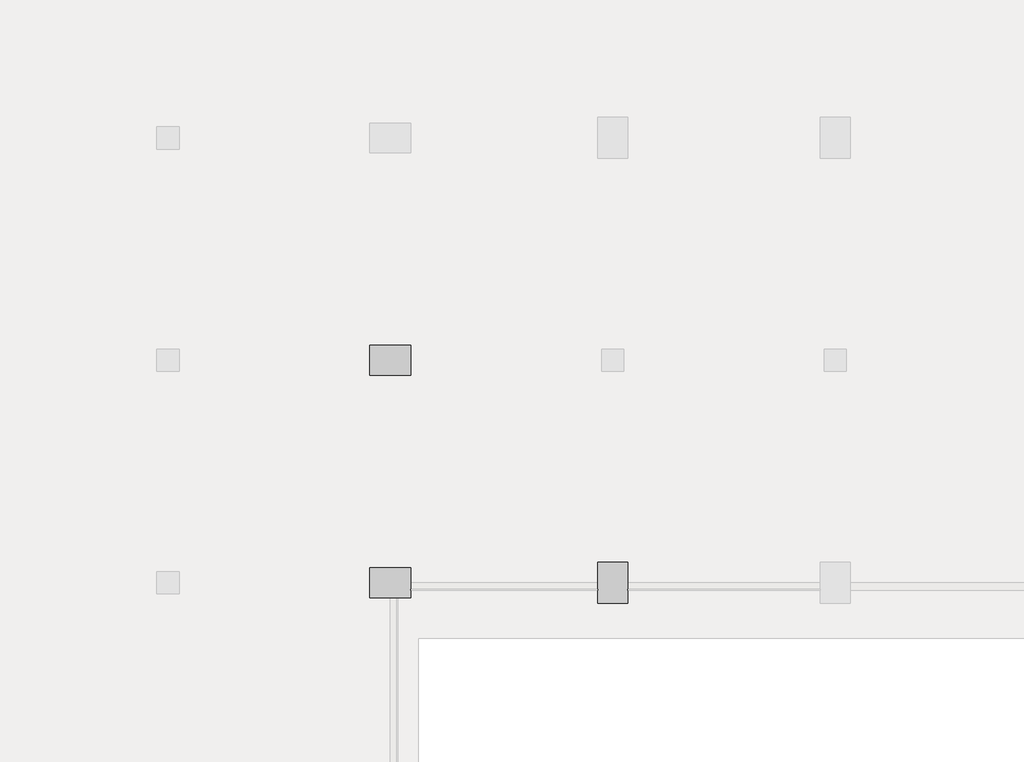
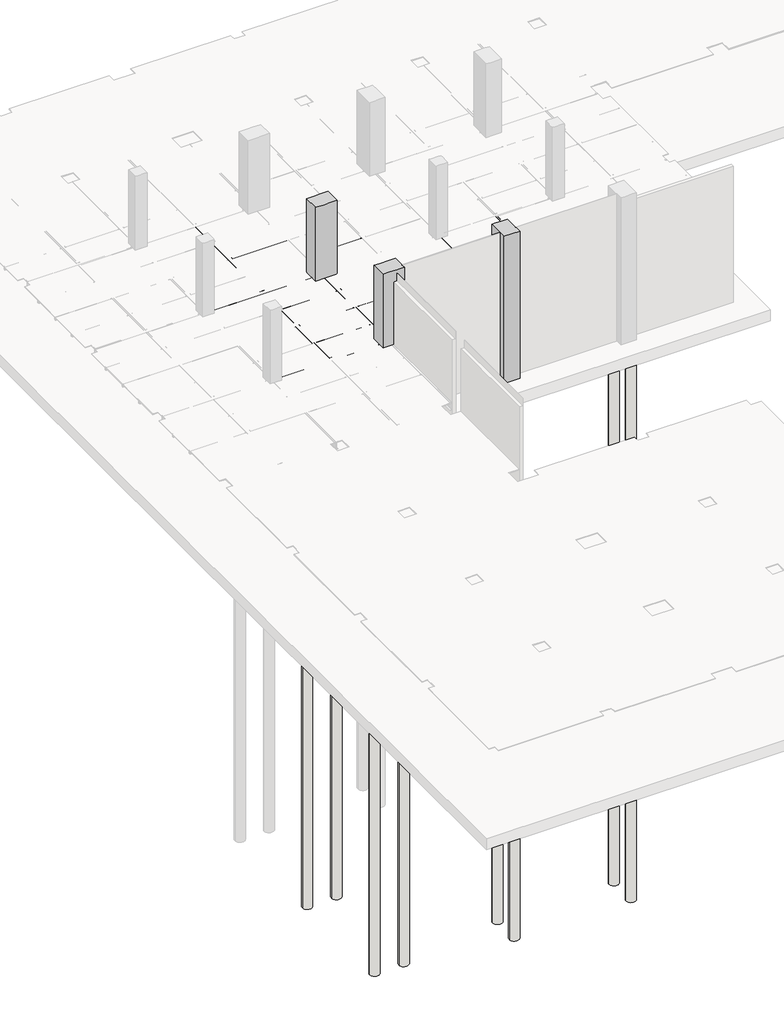
# Not in any storey, part 9 of 16: 28 beams, 8 slabs, 3 columns.
"""IFC4 building model written with IfcOpenShell, lengths in millimetres."""

from ifc_helpers import new_model, si_unit, point, frame, frame_2d, origin, place, context, project, spatial, polyline, circle_curve, trimmed, segment, composite_curve, outline, extrude, faceted_brep, element, save

model = new_model("IFC4")

# Units and contexts
model_context = context("Model", 3, world=origin())
ifc_project = project(units=[si_unit("LENGTHUNIT", "METRE", prefix="MILLI")], contexts=[model_context])

# Site, building
site = spatial("IfcSite", under=ifc_project)
building = spatial("IfcBuilding", under=site)

# Beams
placement = place(None, origin())
element("IfcBeam", 1, ObjectType="Steel Framing_H_KS : H_SB_AR_S02_H-400x200x8x13_BSG1", at=placement, inside=building, context=model_context, shape_type="SweptSolid", body=[
    extrude(outline(composite_curve([segment(polyline([(-23900.0, -4187.0381366), (-23900.0, -4200.0381366), (-24100.0, -4200.0381366), (-24100.0, -4187.0381366), (-24020.0, -4187.0381366)]), True, "CONTINUOUS"), segment(trimmed(circle_curve(frame_2d((-24020.0, -4171.0381366)), 16.0), [point((-24020.0, -4187.0381366))], [point((-24004.0, -4171.0381366))], True, "CARTESIAN"), True, "CONTINUOUS"), segment(polyline([(-24004.0, -4171.0381366), (-24004.0, -3829.0381366)]), True, "CONTINUOUS"), segment(trimmed(circle_curve(frame_2d((-24020.0, -3829.0381366)), 16.0), [point((-24004.0, -3829.0381366))], [point((-24020.0, -3813.0381366))], True, "CARTESIAN"), True, "CONTINUOUS"), segment(polyline([(-24020.0, -3813.0381366), (-24100.0, -3813.0381366), (-24100.0, -3800.0381366), (-23900.0, -3800.0381366), (-23900.0, -3813.0381366), (-23980.0, -3813.0381366)]), True, "CONTINUOUS"), segment(trimmed(circle_curve(frame_2d((-23980.0, -3829.0381366)), 16.0), [point((-23980.0, -3813.0381366))], [point((-23996.0, -3829.0381366))], True, "CARTESIAN"), True, "CONTINUOUS"), segment(polyline([(-23996.0, -3829.0381366), (-23996.0, -4171.0381366)]), True, "CONTINUOUS"), segment(trimmed(circle_curve(frame_2d((-23980.0, -4171.0381366)), 16.0), [point((-23996.0, -4171.0381366))], [point((-23980.0, -4187.0381366))], True, "CARTESIAN"), True, "CONTINUOUS"), segment(polyline([(-23980.0, -4187.0381366), (-23900.0, -4187.0381366)]), True, "CONTINUOUS")], self_intersect=False)), frame((30312.7, 0.0, 0.0), z_axis=(1.0, 0.0, 0.0), x_axis=(0.0, 1.0, 0.0)), (0.0, 0.0, 1.0), 5124.6),
])
element("IfcBeam", 2, ObjectType="Steel Framing_H_KS : H_SB_AR_S02_H-400x200x8x13_BSB1", at=placement, inside=building, context=model_context, shape_type="SweptSolid", body=[
    extrude(outline(composite_curve([segment(polyline([(-4187.0381366, 32900.0), (-4200.0381366, 32900.0), (-4200.0381366, 33100.0), (-4187.0381366, 33100.0), (-4187.0381366, 33020.0)]), True, "CONTINUOUS"), segment(trimmed(circle_curve(frame_2d((-4171.0381366, 33020.0)), 16.0), [point((-4187.0381366, 33020.0))], [point((-4171.0381366, 33004.0))], True, "CARTESIAN"), True, "CONTINUOUS"), segment(polyline([(-4171.0381366, 33004.0), (-3829.0381366, 33004.0)]), True, "CONTINUOUS"), segment(trimmed(circle_curve(frame_2d((-3829.0381366, 33020.0)), 16.0), [point((-3829.0381366, 33004.0))], [point((-3813.0381366, 33020.0))], True, "CARTESIAN"), True, "CONTINUOUS"), segment(polyline([(-3813.0381366, 33020.0), (-3813.0381366, 33100.0), (-3800.0381366, 33100.0), (-3800.0381366, 32900.0), (-3813.0381366, 32900.0), (-3813.0381366, 32980.0)]), True, "CONTINUOUS"), segment(trimmed(circle_curve(frame_2d((-3829.0381366, 32980.0)), 16.0), [point((-3813.0381366, 32980.0))], [point((-3829.0381366, 32996.0))], True, "CARTESIAN"), True, "CONTINUOUS"), segment(polyline([(-3829.0381366, 32996.0), (-4171.0381366, 32996.0)]), True, "CONTINUOUS"), segment(trimmed(circle_curve(frame_2d((-4171.0381366, 32980.0)), 16.0), [point((-4171.0381366, 32996.0))], [point((-4187.0381366, 32980.0))], True, "CARTESIAN"), True, "CONTINUOUS"), segment(polyline([(-4187.0381366, 32980.0), (-4187.0381366, 32900.0)]), True, "CONTINUOUS")], self_intersect=False)), frame((0.0, -23887.3, 0.0), z_axis=(0.0, 1.0, 0.0), x_axis=(0.0, 0.0, 1.0)), (0.0, 0.0, 1.0), 5774.6),
])
element("IfcBeam", 3, ObjectType="Steel Framing_C_KS : H_SB_AR_S02_C-150x75x6.5x10_J1", at=placement, inside=building, context=model_context, shape_type="SweptSolid", body=[
    extrude(outline(composite_curve([segment(polyline([(-20977.2, -3800.0381366), (-20977.2, -3950.0381366), (-21052.2, -3950.0381366)]), True, "CONTINUOUS"), segment(trimmed(circle_curve(frame_2d((-21042.2, -3950.0381366)), 10.0), [point((-21052.2, -3950.0381366))], [point((-21042.2, -3940.0381366))], False, "CARTESIAN"), True, "CONTINUOUS"), segment(polyline([(-21042.2, -3940.0381366), (-20983.7, -3930.7726469), (-20983.7, -3819.3036264), (-21042.2, -3810.0381366)]), True, "CONTINUOUS"), segment(trimmed(circle_curve(frame_2d((-21042.2, -3800.0381366)), 10.0), [point((-21042.2, -3810.0381366))], [point((-21052.2, -3800.0381366))], False, "CARTESIAN"), True, "CONTINUOUS"), segment(polyline([(-21052.2, -3800.0381366), (-20977.2, -3800.0381366)]), True, "CONTINUOUS")], self_intersect=False)), frame((33112.7, 0.0, 0.0), z_axis=(1.0, 0.0, 0.0), x_axis=(0.0, 1.0, 0.0)), (0.0, 0.0, 1.0), 2774.6),
])
element("IfcBeam", 4, ObjectType="Steel Framing_C_KS : H_SB_AR_S02_C-150x75x6.5x10_J1", at=placement, inside=building, context=model_context, shape_type="SweptSolid", body=[
    extrude(outline(composite_curve([segment(polyline([(-22477.2, -3800.0381366), (-22477.2, -3950.0381366), (-22552.2, -3950.0381366)]), True, "CONTINUOUS"), segment(trimmed(circle_curve(frame_2d((-22542.2, -3950.0381366)), 10.0), [point((-22552.2, -3950.0381366))], [point((-22542.2, -3940.0381366))], False, "CARTESIAN"), True, "CONTINUOUS"), segment(polyline([(-22542.2, -3940.0381366), (-22483.7, -3930.7726469), (-22483.7, -3819.3036264), (-22542.2, -3810.0381366)]), True, "CONTINUOUS"), segment(trimmed(circle_curve(frame_2d((-22542.2, -3800.0381366)), 10.0), [point((-22542.2, -3810.0381366))], [point((-22552.2, -3800.0381366))], False, "CARTESIAN"), True, "CONTINUOUS"), segment(polyline([(-22552.2, -3800.0381366), (-22477.2, -3800.0381366)]), True, "CONTINUOUS")], self_intersect=False)), frame((33112.7, 0.0, 0.0), z_axis=(1.0, 0.0, 0.0), x_axis=(0.0, 1.0, 0.0)), (0.0, 0.0, 1.0), 2774.6),
])
element("IfcBeam", 5, ObjectType="Steel Framing_C_KS : H_SB_AR_S02_C-150x75x6.5x10_J1", at=placement, inside=building, context=model_context, shape_type="SweptSolid", body=[
    extrude(outline(composite_curve([segment(polyline([(-22477.2, -3800.0381366), (-22477.2, -3950.0381366), (-22552.2, -3950.0381366)]), True, "CONTINUOUS"), segment(trimmed(circle_curve(frame_2d((-22542.2, -3950.0381366)), 10.0), [point((-22552.2, -3950.0381366))], [point((-22542.2, -3940.0381366))], False, "CARTESIAN"), True, "CONTINUOUS"), segment(polyline([(-22542.2, -3940.0381366), (-22483.7, -3930.7726469), (-22483.7, -3819.3036264), (-22542.2, -3810.0381366)]), True, "CONTINUOUS"), segment(trimmed(circle_curve(frame_2d((-22542.2, -3800.0381366)), 10.0), [point((-22542.2, -3810.0381366))], [point((-22552.2, -3800.0381366))], False, "CARTESIAN"), True, "CONTINUOUS"), segment(polyline([(-22552.2, -3800.0381366), (-22477.2, -3800.0381366)]), True, "CONTINUOUS")], self_intersect=False)), frame((36112.7, 0.0, 0.0), z_axis=(1.0, 0.0, 0.0), x_axis=(0.0, 1.0, 0.0)), (0.0, 0.0, 1.0), 2774.6),
])
element("IfcBeam", 6, ObjectType="Steel Framing_H_KS : H_SB_AR_S02_H-400x200x8x13_BSG1", at=placement, inside=building, context=model_context, shape_type="SweptSolid", body=[
    extrude(outline(composite_curve([segment(polyline([(-29900.0, -4187.0381366), (-29900.0, -4200.0381366), (-30100.0, -4200.0381366), (-30100.0, -4187.0381366), (-30020.0, -4187.0381366)]), True, "CONTINUOUS"), segment(trimmed(circle_curve(frame_2d((-30020.0, -4171.0381366)), 16.0), [point((-30020.0, -4187.0381366))], [point((-30004.0, -4171.0381366))], True, "CARTESIAN"), True, "CONTINUOUS"), segment(polyline([(-30004.0, -4171.0381366), (-30004.0, -3829.0381366)]), True, "CONTINUOUS"), segment(trimmed(circle_curve(frame_2d((-30020.0, -3829.0381366)), 16.0), [point((-30004.0, -3829.0381366))], [point((-30020.0, -3813.0381366))], True, "CARTESIAN"), True, "CONTINUOUS"), segment(polyline([(-30020.0, -3813.0381366), (-30100.0, -3813.0381366), (-30100.0, -3800.0381366), (-29900.0, -3800.0381366), (-29900.0, -3813.0381366), (-29980.0, -3813.0381366)]), True, "CONTINUOUS"), segment(trimmed(circle_curve(frame_2d((-29980.0, -3829.0381366)), 16.0), [point((-29980.0, -3813.0381366))], [point((-29996.0, -3829.0381366))], True, "CARTESIAN"), True, "CONTINUOUS"), segment(polyline([(-29996.0, -3829.0381366), (-29996.0, -4171.0381366)]), True, "CONTINUOUS"), segment(trimmed(circle_curve(frame_2d((-29980.0, -4171.0381366)), 16.0), [point((-29996.0, -4171.0381366))], [point((-29980.0, -4187.0381366))], True, "CARTESIAN"), True, "CONTINUOUS"), segment(polyline([(-29980.0, -4187.0381366), (-29900.0, -4187.0381366)]), True, "CONTINUOUS")], self_intersect=False)), frame((30312.7, 0.0, 0.0), z_axis=(1.0, 0.0, 0.0), x_axis=(0.0, 1.0, 0.0)), (0.0, 0.0, 1.0), 5124.6),
])
element("IfcBeam", 7, ObjectType="Steel Framing_H_KS : H_SB_AR_S02_H-400x200x8x13_BSG2", at=placement, inside=building, context=model_context, shape_type="SweptSolid", body=[
    extrude(outline(composite_curve([segment(polyline([(-4187.0381366, 35900.0), (-4200.0381366, 35900.0), (-4200.0381366, 36100.0), (-4187.0381366, 36100.0), (-4187.0381366, 36020.0)]), True, "CONTINUOUS"), segment(trimmed(circle_curve(frame_2d((-4171.0381366, 36020.0)), 16.0), [point((-4187.0381366, 36020.0))], [point((-4171.0381366, 36004.0))], True, "CARTESIAN"), True, "CONTINUOUS"), segment(polyline([(-4171.0381366, 36004.0), (-3829.0381366, 36004.0)]), True, "CONTINUOUS"), segment(trimmed(circle_curve(frame_2d((-3829.0381366, 36020.0)), 16.0), [point((-3829.0381366, 36004.0))], [point((-3813.0381366, 36020.0))], True, "CARTESIAN"), True, "CONTINUOUS"), segment(polyline([(-3813.0381366, 36020.0), (-3813.0381366, 36100.0), (-3800.0381366, 36100.0), (-3800.0381366, 35900.0), (-3813.0381366, 35900.0), (-3813.0381366, 35980.0)]), True, "CONTINUOUS"), segment(trimmed(circle_curve(frame_2d((-3829.0381366, 35980.0)), 16.0), [point((-3813.0381366, 35980.0))], [point((-3829.0381366, 35996.0))], True, "CARTESIAN"), True, "CONTINUOUS"), segment(polyline([(-3829.0381366, 35996.0), (-4171.0381366, 35996.0)]), True, "CONTINUOUS"), segment(trimmed(circle_curve(frame_2d((-4171.0381366, 35980.0)), 16.0), [point((-4171.0381366, 35996.0))], [point((-4187.0381366, 35980.0))], True, "CARTESIAN"), True, "CONTINUOUS"), segment(polyline([(-4187.0381366, 35980.0), (-4187.0381366, 35900.0)]), True, "CONTINUOUS")], self_intersect=False)), frame((0.0, -29587.3, 0.0), z_axis=(0.0, 1.0, 0.0), x_axis=(0.0, 0.0, 1.0)), (0.0, 0.0, 1.0), 5174.6),
])
element("IfcBeam", 8, ObjectType="Steel Framing_H_KS : H_SB_AR_S02_H-400x200x8x13_BSB1", at=placement, inside=building, context=model_context, shape_type="SweptSolid", body=[
    extrude(outline(composite_curve([segment(polyline([(-4187.0381366, 32900.0), (-4200.0381366, 32900.0), (-4200.0381366, 33100.0), (-4187.0381366, 33100.0), (-4187.0381366, 33020.0)]), True, "CONTINUOUS"), segment(trimmed(circle_curve(frame_2d((-4171.0381366, 33020.0)), 16.0), [point((-4187.0381366, 33020.0))], [point((-4171.0381366, 33004.0))], True, "CARTESIAN"), True, "CONTINUOUS"), segment(polyline([(-4171.0381366, 33004.0), (-3829.0381366, 33004.0)]), True, "CONTINUOUS"), segment(trimmed(circle_curve(frame_2d((-3829.0381366, 33020.0)), 16.0), [point((-3829.0381366, 33004.0))], [point((-3813.0381366, 33020.0))], True, "CARTESIAN"), True, "CONTINUOUS"), segment(polyline([(-3813.0381366, 33020.0), (-3813.0381366, 33100.0), (-3800.0381366, 33100.0), (-3800.0381366, 32900.0), (-3813.0381366, 32900.0), (-3813.0381366, 32980.0)]), True, "CONTINUOUS"), segment(trimmed(circle_curve(frame_2d((-3829.0381366, 32980.0)), 16.0), [point((-3813.0381366, 32980.0))], [point((-3829.0381366, 32996.0))], True, "CARTESIAN"), True, "CONTINUOUS"), segment(polyline([(-3829.0381366, 32996.0), (-4171.0381366, 32996.0)]), True, "CONTINUOUS"), segment(trimmed(circle_curve(frame_2d((-4171.0381366, 32980.0)), 16.0), [point((-4171.0381366, 32996.0))], [point((-4187.0381366, 32980.0))], True, "CARTESIAN"), True, "CONTINUOUS"), segment(polyline([(-4187.0381366, 32980.0), (-4187.0381366, 32900.0)]), True, "CONTINUOUS")], self_intersect=False)), frame((0.0, -29887.3, 0.0), z_axis=(0.0, 1.0, 0.0), x_axis=(0.0, 0.0, 1.0)), (0.0, 0.0, 1.0), 5774.6),
])
element("IfcBeam", 9, ObjectType="Steel Framing_C_KS : H_SB_AR_S02_C-150x75x6.5x10_J1", at=placement, inside=building, context=model_context, shape_type="SweptSolid", body=[
    extrude(outline(composite_curve([segment(polyline([(-26977.2, -3800.0381366), (-26977.2, -3950.0381366), (-27052.2, -3950.0381366)]), True, "CONTINUOUS"), segment(trimmed(circle_curve(frame_2d((-27042.2, -3950.0381366)), 10.0), [point((-27052.2, -3950.0381366))], [point((-27042.2, -3940.0381366))], False, "CARTESIAN"), True, "CONTINUOUS"), segment(polyline([(-27042.2, -3940.0381366), (-26983.7, -3930.7726469), (-26983.7, -3819.3036264), (-27042.2, -3810.0381366)]), True, "CONTINUOUS"), segment(trimmed(circle_curve(frame_2d((-27042.2, -3800.0381366)), 10.0), [point((-27042.2, -3810.0381366))], [point((-27052.2, -3800.0381366))], False, "CARTESIAN"), True, "CONTINUOUS"), segment(polyline([(-27052.2, -3800.0381366), (-26977.2, -3800.0381366)]), True, "CONTINUOUS")], self_intersect=False)), frame((33112.7, 0.0, 0.0), z_axis=(1.0, 0.0, 0.0), x_axis=(0.0, 1.0, 0.0)), (0.0, 0.0, 1.0), 2774.6),
])
element("IfcBeam", 10, ObjectType="Steel Framing_C_KS : H_SB_AR_S02_C-150x75x6.5x10_J1", at=placement, inside=building, context=model_context, shape_type="SweptSolid", body=[
    extrude(outline(composite_curve([segment(polyline([(-28477.2, -3800.0381366), (-28477.2, -3950.0381366), (-28552.2, -3950.0381366)]), True, "CONTINUOUS"), segment(trimmed(circle_curve(frame_2d((-28542.2, -3950.0381366)), 10.0), [point((-28552.2, -3950.0381366))], [point((-28542.2, -3940.0381366))], False, "CARTESIAN"), True, "CONTINUOUS"), segment(polyline([(-28542.2, -3940.0381366), (-28483.7, -3930.7726469), (-28483.7, -3819.3036264), (-28542.2, -3810.0381366)]), True, "CONTINUOUS"), segment(trimmed(circle_curve(frame_2d((-28542.2, -3800.0381366)), 10.0), [point((-28542.2, -3810.0381366))], [point((-28552.2, -3800.0381366))], False, "CARTESIAN"), True, "CONTINUOUS"), segment(polyline([(-28552.2, -3800.0381366), (-28477.2, -3800.0381366)]), True, "CONTINUOUS")], self_intersect=False)), frame((33112.7, 0.0, 0.0), z_axis=(1.0, 0.0, 0.0), x_axis=(0.0, 1.0, 0.0)), (0.0, 0.0, 1.0), 2774.6),
])
element("IfcBeam", 11, ObjectType="Steel Framing_C_KS : H_SB_AR_S02_C-150x75x6.5x10_J1", at=placement, inside=building, context=model_context, shape_type="SweptSolid", body=[
    extrude(outline(composite_curve([segment(polyline([(-25477.2, -3800.0381366), (-25477.2, -3950.0381366), (-25552.2, -3950.0381366)]), True, "CONTINUOUS"), segment(trimmed(circle_curve(frame_2d((-25542.2, -3950.0381366)), 10.0), [point((-25552.2, -3950.0381366))], [point((-25542.2, -3940.0381366))], False, "CARTESIAN"), True, "CONTINUOUS"), segment(polyline([(-25542.2, -3940.0381366), (-25483.7, -3930.7726469), (-25483.7, -3819.3036264), (-25542.2, -3810.0381366)]), True, "CONTINUOUS"), segment(trimmed(circle_curve(frame_2d((-25542.2, -3800.0381366)), 10.0), [point((-25542.2, -3810.0381366))], [point((-25552.2, -3800.0381366))], False, "CARTESIAN"), True, "CONTINUOUS"), segment(polyline([(-25552.2, -3800.0381366), (-25477.2, -3800.0381366)]), True, "CONTINUOUS")], self_intersect=False)), frame((33112.7, 0.0, 0.0), z_axis=(1.0, 0.0, 0.0), x_axis=(0.0, 1.0, 0.0)), (0.0, 0.0, 1.0), 2774.6),
])
element("IfcBeam", 12, ObjectType="Steel Framing_H_KS : H_SB_AR_S02_H-400x200x8x13_BSG1", at=placement, inside=building, context=model_context, shape_type="SweptSolid", body=[
    extrude(outline(composite_curve([segment(polyline([(-29900.0, -4187.0381366), (-29900.0, -4200.0381366), (-30100.0, -4200.0381366), (-30100.0, -4187.0381366), (-30020.0, -4187.0381366)]), True, "CONTINUOUS"), segment(trimmed(circle_curve(frame_2d((-30020.0, -4171.0381366)), 16.0), [point((-30020.0, -4187.0381366))], [point((-30004.0, -4171.0381366))], True, "CARTESIAN"), True, "CONTINUOUS"), segment(polyline([(-30004.0, -4171.0381366), (-30004.0, -3829.0381366)]), True, "CONTINUOUS"), segment(trimmed(circle_curve(frame_2d((-30020.0, -3829.0381366)), 16.0), [point((-30004.0, -3829.0381366))], [point((-30020.0, -3813.0381366))], True, "CARTESIAN"), True, "CONTINUOUS"), segment(polyline([(-30020.0, -3813.0381366), (-30100.0, -3813.0381366), (-30100.0, -3800.0381366), (-29900.0, -3800.0381366), (-29900.0, -3813.0381366), (-29980.0, -3813.0381366)]), True, "CONTINUOUS"), segment(trimmed(circle_curve(frame_2d((-29980.0, -3829.0381366)), 16.0), [point((-29980.0, -3813.0381366))], [point((-29996.0, -3829.0381366))], True, "CARTESIAN"), True, "CONTINUOUS"), segment(polyline([(-29996.0, -3829.0381366), (-29996.0, -4171.0381366)]), True, "CONTINUOUS"), segment(trimmed(circle_curve(frame_2d((-29980.0, -4171.0381366)), 16.0), [point((-29996.0, -4171.0381366))], [point((-29980.0, -4187.0381366))], True, "CARTESIAN"), True, "CONTINUOUS"), segment(polyline([(-29980.0, -4187.0381366), (-29900.0, -4187.0381366)]), True, "CONTINUOUS")], self_intersect=False)), frame((36562.7, 0.0, 0.0), z_axis=(1.0, 0.0, 0.0), x_axis=(0.0, 1.0, 0.0)), (0.0, 0.0, 1.0), 5024.6),
])
element("IfcBeam", 13, ObjectType="Steel Framing_H_KS : H_SB_AR_S02_H-400x200x8x13_BSG2", at=placement, inside=building, context=model_context, shape_type="SweptSolid", body=[
    extrude(outline(composite_curve([segment(polyline([(-4187.0381366, 41900.0), (-4200.0381366, 41900.0), (-4200.0381366, 42100.0), (-4187.0381366, 42100.0), (-4187.0381366, 42020.0)]), True, "CONTINUOUS"), segment(trimmed(circle_curve(frame_2d((-4171.0381366, 42020.0)), 16.0), [point((-4187.0381366, 42020.0))], [point((-4171.0381366, 42004.0))], True, "CARTESIAN"), True, "CONTINUOUS"), segment(polyline([(-4171.0381366, 42004.0), (-3829.0381366, 42004.0)]), True, "CONTINUOUS"), segment(trimmed(circle_curve(frame_2d((-3829.0381366, 42020.0)), 16.0), [point((-3829.0381366, 42004.0))], [point((-3813.0381366, 42020.0))], True, "CARTESIAN"), True, "CONTINUOUS"), segment(polyline([(-3813.0381366, 42020.0), (-3813.0381366, 42100.0), (-3800.0381366, 42100.0), (-3800.0381366, 41900.0), (-3813.0381366, 41900.0), (-3813.0381366, 41980.0)]), True, "CONTINUOUS"), segment(trimmed(circle_curve(frame_2d((-3829.0381366, 41980.0)), 16.0), [point((-3813.0381366, 41980.0))], [point((-3829.0381366, 41996.0))], True, "CARTESIAN"), True, "CONTINUOUS"), segment(polyline([(-3829.0381366, 41996.0), (-4171.0381366, 41996.0)]), True, "CONTINUOUS"), segment(trimmed(circle_curve(frame_2d((-4171.0381366, 41980.0)), 16.0), [point((-4171.0381366, 41996.0))], [point((-4187.0381366, 41980.0))], True, "CARTESIAN"), True, "CONTINUOUS"), segment(polyline([(-4187.0381366, 41980.0), (-4187.0381366, 41900.0)]), True, "CONTINUOUS")], self_intersect=False)), frame((0.0, -29437.3, 0.0), z_axis=(0.0, 1.0, 0.0), x_axis=(0.0, 0.0, 1.0)), (0.0, 0.0, 1.0), 5124.6),
])
element("IfcBeam", 14, ObjectType="Steel Framing_H_KS : H_SB_AR_S02_H-400x200x8x13_BSB1", at=placement, inside=building, context=model_context, shape_type="SweptSolid", body=[
    extrude(outline(composite_curve([segment(polyline([(-4187.0381366, 38900.0), (-4200.0381366, 38900.0), (-4200.0381366, 39100.0), (-4187.0381366, 39100.0), (-4187.0381366, 39020.0)]), True, "CONTINUOUS"), segment(trimmed(circle_curve(frame_2d((-4171.0381366, 39020.0)), 16.0), [point((-4187.0381366, 39020.0))], [point((-4171.0381366, 39004.0))], True, "CARTESIAN"), True, "CONTINUOUS"), segment(polyline([(-4171.0381366, 39004.0), (-3829.0381366, 39004.0)]), True, "CONTINUOUS"), segment(trimmed(circle_curve(frame_2d((-3829.0381366, 39020.0)), 16.0), [point((-3829.0381366, 39004.0))], [point((-3813.0381366, 39020.0))], True, "CARTESIAN"), True, "CONTINUOUS"), segment(polyline([(-3813.0381366, 39020.0), (-3813.0381366, 39100.0), (-3800.0381366, 39100.0), (-3800.0381366, 38900.0), (-3813.0381366, 38900.0), (-3813.0381366, 38980.0)]), True, "CONTINUOUS"), segment(trimmed(circle_curve(frame_2d((-3829.0381366, 38980.0)), 16.0), [point((-3813.0381366, 38980.0))], [point((-3829.0381366, 38996.0))], True, "CARTESIAN"), True, "CONTINUOUS"), segment(polyline([(-3829.0381366, 38996.0), (-4171.0381366, 38996.0)]), True, "CONTINUOUS"), segment(trimmed(circle_curve(frame_2d((-4171.0381366, 38980.0)), 16.0), [point((-4171.0381366, 38996.0))], [point((-4187.0381366, 38980.0))], True, "CARTESIAN"), True, "CONTINUOUS"), segment(polyline([(-4187.0381366, 38980.0), (-4187.0381366, 38900.0)]), True, "CONTINUOUS")], self_intersect=False)), frame((0.0, -29887.3, 0.0), z_axis=(0.0, 1.0, 0.0), x_axis=(0.0, 0.0, 1.0)), (0.0, 0.0, 1.0), 5774.6),
])
element("IfcBeam", 15, ObjectType="Steel Framing_C_KS : H_SB_AR_S02_C-150x75x6.5x10_J1", at=placement, inside=building, context=model_context, shape_type="SweptSolid", body=[
    extrude(outline(composite_curve([segment(polyline([(-26977.2, -3800.0381366), (-26977.2, -3950.0381366), (-27052.2, -3950.0381366)]), True, "CONTINUOUS"), segment(trimmed(circle_curve(frame_2d((-27042.2, -3950.0381366)), 10.0), [point((-27052.2, -3950.0381366))], [point((-27042.2, -3940.0381366))], False, "CARTESIAN"), True, "CONTINUOUS"), segment(polyline([(-27042.2, -3940.0381366), (-26983.7, -3930.7726469), (-26983.7, -3819.3036264), (-27042.2, -3810.0381366)]), True, "CONTINUOUS"), segment(trimmed(circle_curve(frame_2d((-27042.2, -3800.0381366)), 10.0), [point((-27042.2, -3810.0381366))], [point((-27052.2, -3800.0381366))], False, "CARTESIAN"), True, "CONTINUOUS"), segment(polyline([(-27052.2, -3800.0381366), (-26977.2, -3800.0381366)]), True, "CONTINUOUS")], self_intersect=False)), frame((36112.7, 0.0, 0.0), z_axis=(1.0, 0.0, 0.0), x_axis=(0.0, 1.0, 0.0)), (0.0, 0.0, 1.0), 2774.6),
])
element("IfcBeam", 16, ObjectType="Steel Framing_C_KS : H_SB_AR_S02_C-150x75x6.5x10_J1", at=placement, inside=building, context=model_context, shape_type="SweptSolid", body=[
    extrude(outline(composite_curve([segment(polyline([(-28477.2, -3800.0381366), (-28477.2, -3950.0381366), (-28552.2, -3950.0381366)]), True, "CONTINUOUS"), segment(trimmed(circle_curve(frame_2d((-28542.2, -3950.0381366)), 10.0), [point((-28552.2, -3950.0381366))], [point((-28542.2, -3940.0381366))], False, "CARTESIAN"), True, "CONTINUOUS"), segment(polyline([(-28542.2, -3940.0381366), (-28483.7, -3930.7726469), (-28483.7, -3819.3036264), (-28542.2, -3810.0381366)]), True, "CONTINUOUS"), segment(trimmed(circle_curve(frame_2d((-28542.2, -3800.0381366)), 10.0), [point((-28542.2, -3810.0381366))], [point((-28552.2, -3800.0381366))], False, "CARTESIAN"), True, "CONTINUOUS"), segment(polyline([(-28552.2, -3800.0381366), (-28477.2, -3800.0381366)]), True, "CONTINUOUS")], self_intersect=False)), frame((36112.7, 0.0, 0.0), z_axis=(1.0, 0.0, 0.0), x_axis=(0.0, 1.0, 0.0)), (0.0, 0.0, 1.0), 2774.6),
])
element("IfcBeam", 17, ObjectType="Steel Framing_C_KS : H_SB_AR_S02_C-150x75x6.5x10_J1", at=placement, inside=building, context=model_context, shape_type="SweptSolid", body=[
    extrude(outline(composite_curve([segment(polyline([(-25477.2, -3800.0381366), (-25477.2, -3950.0381366), (-25552.2, -3950.0381366)]), True, "CONTINUOUS"), segment(trimmed(circle_curve(frame_2d((-25542.2, -3950.0381366)), 10.0), [point((-25552.2, -3950.0381366))], [point((-25542.2, -3940.0381366))], False, "CARTESIAN"), True, "CONTINUOUS"), segment(polyline([(-25542.2, -3940.0381366), (-25483.7, -3930.7726469), (-25483.7, -3819.3036264), (-25542.2, -3810.0381366)]), True, "CONTINUOUS"), segment(trimmed(circle_curve(frame_2d((-25542.2, -3800.0381366)), 10.0), [point((-25542.2, -3810.0381366))], [point((-25552.2, -3800.0381366))], False, "CARTESIAN"), True, "CONTINUOUS"), segment(polyline([(-25552.2, -3800.0381366), (-25477.2, -3800.0381366)]), True, "CONTINUOUS")], self_intersect=False)), frame((36112.7, 0.0, 0.0), z_axis=(1.0, 0.0, 0.0), x_axis=(0.0, 1.0, 0.0)), (0.0, 0.0, 1.0), 2774.6),
])
element("IfcBeam", 18, ObjectType="Steel Framing_C_KS : H_SB_AR_S02_C-150x75x6.5x10_J1", at=placement, inside=building, context=model_context, shape_type="SweptSolid", body=[
    extrude(outline(composite_curve([segment(polyline([(-26977.2, -3800.0381366), (-26977.2, -3950.0381366), (-27052.2, -3950.0381366)]), True, "CONTINUOUS"), segment(trimmed(circle_curve(frame_2d((-27042.2, -3950.0381366)), 10.0), [point((-27052.2, -3950.0381366))], [point((-27042.2, -3940.0381366))], False, "CARTESIAN"), True, "CONTINUOUS"), segment(polyline([(-27042.2, -3940.0381366), (-26983.7, -3930.7726469), (-26983.7, -3819.3036264), (-27042.2, -3810.0381366)]), True, "CONTINUOUS"), segment(trimmed(circle_curve(frame_2d((-27042.2, -3800.0381366)), 10.0), [point((-27042.2, -3810.0381366))], [point((-27052.2, -3800.0381366))], False, "CARTESIAN"), True, "CONTINUOUS"), segment(polyline([(-27052.2, -3800.0381366), (-26977.2, -3800.0381366)]), True, "CONTINUOUS")], self_intersect=False)), frame((39112.7, 0.0, 0.0), z_axis=(1.0, 0.0, 0.0), x_axis=(0.0, 1.0, 0.0)), (0.0, 0.0, 1.0), 2774.6),
])
element("IfcBeam", 19, ObjectType="Steel Framing_C_KS : H_SB_AR_S02_C-150x75x6.5x10_J1", at=placement, inside=building, context=model_context, shape_type="SweptSolid", body=[
    extrude(outline(composite_curve([segment(polyline([(-28477.2, -3800.0381366), (-28477.2, -3950.0381366), (-28552.2, -3950.0381366)]), True, "CONTINUOUS"), segment(trimmed(circle_curve(frame_2d((-28542.2, -3950.0381366)), 10.0), [point((-28552.2, -3950.0381366))], [point((-28542.2, -3940.0381366))], False, "CARTESIAN"), True, "CONTINUOUS"), segment(polyline([(-28542.2, -3940.0381366), (-28483.7, -3930.7726469), (-28483.7, -3819.3036264), (-28542.2, -3810.0381366)]), True, "CONTINUOUS"), segment(trimmed(circle_curve(frame_2d((-28542.2, -3800.0381366)), 10.0), [point((-28542.2, -3810.0381366))], [point((-28552.2, -3800.0381366))], False, "CARTESIAN"), True, "CONTINUOUS"), segment(polyline([(-28552.2, -3800.0381366), (-28477.2, -3800.0381366)]), True, "CONTINUOUS")], self_intersect=False)), frame((39112.7, 0.0, 0.0), z_axis=(1.0, 0.0, 0.0), x_axis=(0.0, 1.0, 0.0)), (0.0, 0.0, 1.0), 2774.6),
])
element("IfcBeam", 20, ObjectType="Steel Framing_C_KS : H_SB_AR_S02_C-150x75x6.5x10_J1", at=placement, inside=building, context=model_context, shape_type="SweptSolid", body=[
    extrude(outline(composite_curve([segment(polyline([(-25477.2, -3800.0381366), (-25477.2, -3950.0381366), (-25552.2, -3950.0381366)]), True, "CONTINUOUS"), segment(trimmed(circle_curve(frame_2d((-25542.2, -3950.0381366)), 10.0), [point((-25552.2, -3950.0381366))], [point((-25542.2, -3940.0381366))], False, "CARTESIAN"), True, "CONTINUOUS"), segment(polyline([(-25542.2, -3940.0381366), (-25483.7, -3930.7726469), (-25483.7, -3819.3036264), (-25542.2, -3810.0381366)]), True, "CONTINUOUS"), segment(trimmed(circle_curve(frame_2d((-25542.2, -3800.0381366)), 10.0), [point((-25542.2, -3810.0381366))], [point((-25552.2, -3800.0381366))], False, "CARTESIAN"), True, "CONTINUOUS"), segment(polyline([(-25552.2, -3800.0381366), (-25477.2, -3800.0381366)]), True, "CONTINUOUS")], self_intersect=False)), frame((39112.7, 0.0, 0.0), z_axis=(1.0, 0.0, 0.0), x_axis=(0.0, 1.0, 0.0)), (0.0, 0.0, 1.0), 2774.6),
])
element("IfcBeam", 21, ObjectType="Steel Framing_H_KS : H_SB_AR_S02_H-400x200x8x13_BSG1", at=placement, inside=building, context=model_context, shape_type="SweptSolid", body=[
    extrude(outline(composite_curve([segment(polyline([(-29900.0, -4187.0381366), (-29900.0, -4200.0381366), (-30100.0, -4200.0381366), (-30100.0, -4187.0381366), (-30020.0, -4187.0381366)]), True, "CONTINUOUS"), segment(trimmed(circle_curve(frame_2d((-30020.0, -4171.0381366)), 16.0), [point((-30020.0, -4187.0381366))], [point((-30004.0, -4171.0381366))], True, "CARTESIAN"), True, "CONTINUOUS"), segment(polyline([(-30004.0, -4171.0381366), (-30004.0, -3829.0381366)]), True, "CONTINUOUS"), segment(trimmed(circle_curve(frame_2d((-30020.0, -3829.0381366)), 16.0), [point((-30004.0, -3829.0381366))], [point((-30020.0, -3813.0381366))], True, "CARTESIAN"), True, "CONTINUOUS"), segment(polyline([(-30020.0, -3813.0381366), (-30100.0, -3813.0381366), (-30100.0, -3800.0381366), (-29900.0, -3800.0381366), (-29900.0, -3813.0381366), (-29980.0, -3813.0381366)]), True, "CONTINUOUS"), segment(trimmed(circle_curve(frame_2d((-29980.0, -3829.0381366)), 16.0), [point((-29980.0, -3813.0381366))], [point((-29996.0, -3829.0381366))], True, "CARTESIAN"), True, "CONTINUOUS"), segment(polyline([(-29996.0, -3829.0381366), (-29996.0, -4171.0381366)]), True, "CONTINUOUS"), segment(trimmed(circle_curve(frame_2d((-29980.0, -4171.0381366)), 16.0), [point((-29996.0, -4171.0381366))], [point((-29980.0, -4187.0381366))], True, "CARTESIAN"), True, "CONTINUOUS"), segment(polyline([(-29980.0, -4187.0381366), (-29900.0, -4187.0381366)]), True, "CONTINUOUS")], self_intersect=False)), frame((42412.7, 0.0, 0.0), z_axis=(1.0, 0.0, 0.0), x_axis=(0.0, 1.0, 0.0)), (0.0, 0.0, 1.0), 5174.6),
])
element("IfcBeam", 22, ObjectType="Steel Framing_H_KS : H_SB_AR_S02_H-400x200x8x13_BSB1", at=placement, inside=building, context=model_context, shape_type="SweptSolid", body=[
    extrude(outline(composite_curve([segment(polyline([(-4187.0381366, 44900.0), (-4200.0381366, 44900.0), (-4200.0381366, 45100.0), (-4187.0381366, 45100.0), (-4187.0381366, 45020.0)]), True, "CONTINUOUS"), segment(trimmed(circle_curve(frame_2d((-4171.0381366, 45020.0)), 16.0), [point((-4187.0381366, 45020.0))], [point((-4171.0381366, 45004.0))], True, "CARTESIAN"), True, "CONTINUOUS"), segment(polyline([(-4171.0381366, 45004.0), (-3829.0381366, 45004.0)]), True, "CONTINUOUS"), segment(trimmed(circle_curve(frame_2d((-3829.0381366, 45020.0)), 16.0), [point((-3829.0381366, 45004.0))], [point((-3813.0381366, 45020.0))], True, "CARTESIAN"), True, "CONTINUOUS"), segment(polyline([(-3813.0381366, 45020.0), (-3813.0381366, 45100.0), (-3800.0381366, 45100.0), (-3800.0381366, 44900.0), (-3813.0381366, 44900.0), (-3813.0381366, 44980.0)]), True, "CONTINUOUS"), segment(trimmed(circle_curve(frame_2d((-3829.0381366, 44980.0)), 16.0), [point((-3813.0381366, 44980.0))], [point((-3829.0381366, 44996.0))], True, "CARTESIAN"), True, "CONTINUOUS"), segment(polyline([(-3829.0381366, 44996.0), (-4171.0381366, 44996.0)]), True, "CONTINUOUS"), segment(trimmed(circle_curve(frame_2d((-4171.0381366, 44980.0)), 16.0), [point((-4171.0381366, 44996.0))], [point((-4187.0381366, 44980.0))], True, "CARTESIAN"), True, "CONTINUOUS"), segment(polyline([(-4187.0381366, 44980.0), (-4187.0381366, 44900.0)]), True, "CONTINUOUS")], self_intersect=False)), frame((0.0, -29887.3, 0.0), z_axis=(0.0, 1.0, 0.0), x_axis=(0.0, 0.0, 1.0)), (0.0, 0.0, 1.0), 5774.6),
])
element("IfcBeam", 23, ObjectType="Steel Framing_C_KS : H_SB_AR_S02_C-150x75x6.5x10_J1", at=placement, inside=building, context=model_context, shape_type="SweptSolid", body=[
    extrude(outline(composite_curve([segment(polyline([(-26977.2, -3800.0381366), (-26977.2, -3950.0381366), (-27052.2, -3950.0381366)]), True, "CONTINUOUS"), segment(trimmed(circle_curve(frame_2d((-27042.2, -3950.0381366)), 10.0), [point((-27052.2, -3950.0381366))], [point((-27042.2, -3940.0381366))], False, "CARTESIAN"), True, "CONTINUOUS"), segment(polyline([(-27042.2, -3940.0381366), (-26983.7, -3930.7726469), (-26983.7, -3819.3036264), (-27042.2, -3810.0381366)]), True, "CONTINUOUS"), segment(trimmed(circle_curve(frame_2d((-27042.2, -3800.0381366)), 10.0), [point((-27042.2, -3810.0381366))], [point((-27052.2, -3800.0381366))], False, "CARTESIAN"), True, "CONTINUOUS"), segment(polyline([(-27052.2, -3800.0381366), (-26977.2, -3800.0381366)]), True, "CONTINUOUS")], self_intersect=False)), frame((42112.7, 0.0, 0.0), z_axis=(1.0, 0.0, 0.0), x_axis=(0.0, 1.0, 0.0)), (0.0, 0.0, 1.0), 2774.6),
])
element("IfcBeam", 24, ObjectType="Steel Framing_C_KS : H_SB_AR_S02_C-150x75x6.5x10_J1", at=placement, inside=building, context=model_context, shape_type="SweptSolid", body=[
    extrude(outline(composite_curve([segment(polyline([(-28477.2, -3800.0381366), (-28477.2, -3950.0381366), (-28552.2, -3950.0381366)]), True, "CONTINUOUS"), segment(trimmed(circle_curve(frame_2d((-28542.2, -3950.0381366)), 10.0), [point((-28552.2, -3950.0381366))], [point((-28542.2, -3940.0381366))], False, "CARTESIAN"), True, "CONTINUOUS"), segment(polyline([(-28542.2, -3940.0381366), (-28483.7, -3930.7726469), (-28483.7, -3819.3036264), (-28542.2, -3810.0381366)]), True, "CONTINUOUS"), segment(trimmed(circle_curve(frame_2d((-28542.2, -3800.0381366)), 10.0), [point((-28542.2, -3810.0381366))], [point((-28552.2, -3800.0381366))], False, "CARTESIAN"), True, "CONTINUOUS"), segment(polyline([(-28552.2, -3800.0381366), (-28477.2, -3800.0381366)]), True, "CONTINUOUS")], self_intersect=False)), frame((42112.7, 0.0, 0.0), z_axis=(1.0, 0.0, 0.0), x_axis=(0.0, 1.0, 0.0)), (0.0, 0.0, 1.0), 2774.6),
])
element("IfcBeam", 25, ObjectType="Steel Framing_C_KS : H_SB_AR_S02_C-150x75x6.5x10_J1", at=placement, inside=building, context=model_context, shape_type="SweptSolid", body=[
    extrude(outline(composite_curve([segment(polyline([(-25477.2, -3800.0381366), (-25477.2, -3950.0381366), (-25552.2, -3950.0381366)]), True, "CONTINUOUS"), segment(trimmed(circle_curve(frame_2d((-25542.2, -3950.0381366)), 10.0), [point((-25552.2, -3950.0381366))], [point((-25542.2, -3940.0381366))], False, "CARTESIAN"), True, "CONTINUOUS"), segment(polyline([(-25542.2, -3940.0381366), (-25483.7, -3930.7726469), (-25483.7, -3819.3036264), (-25542.2, -3810.0381366)]), True, "CONTINUOUS"), segment(trimmed(circle_curve(frame_2d((-25542.2, -3800.0381366)), 10.0), [point((-25542.2, -3810.0381366))], [point((-25552.2, -3800.0381366))], False, "CARTESIAN"), True, "CONTINUOUS"), segment(polyline([(-25552.2, -3800.0381366), (-25477.2, -3800.0381366)]), True, "CONTINUOUS")], self_intersect=False)), frame((42112.7, 0.0, 0.0), z_axis=(1.0, 0.0, 0.0), x_axis=(0.0, 1.0, 0.0)), (0.0, 0.0, 1.0), 2774.6),
])
element("IfcBeam", 26, ObjectType="Steel Framing_C_KS : H_SB_AR_S02_C-150x75x6.5x10_J1", at=placement, inside=building, context=model_context, shape_type="SweptSolid", body=[
    extrude(outline(composite_curve([segment(polyline([(-26977.2, -3800.0381366), (-26977.2, -3950.0381366), (-27052.2, -3950.0381366)]), True, "CONTINUOUS"), segment(trimmed(circle_curve(frame_2d((-27042.2, -3950.0381366)), 10.0), [point((-27052.2, -3950.0381366))], [point((-27042.2, -3940.0381366))], False, "CARTESIAN"), True, "CONTINUOUS"), segment(polyline([(-27042.2, -3940.0381366), (-26983.7, -3930.7726469), (-26983.7, -3819.3036264), (-27042.2, -3810.0381366)]), True, "CONTINUOUS"), segment(trimmed(circle_curve(frame_2d((-27042.2, -3800.0381366)), 10.0), [point((-27042.2, -3810.0381366))], [point((-27052.2, -3800.0381366))], False, "CARTESIAN"), True, "CONTINUOUS"), segment(polyline([(-27052.2, -3800.0381366), (-26977.2, -3800.0381366)]), True, "CONTINUOUS")], self_intersect=False)), frame((45112.7, 0.0, 0.0), z_axis=(1.0, 0.0, 0.0), x_axis=(0.0, 1.0, 0.0)), (0.0, 0.0, 1.0), 2774.6),
])
element("IfcBeam", 27, ObjectType="Steel Framing_C_KS : H_SB_AR_S02_C-150x75x6.5x10_J1", at=placement, inside=building, context=model_context, shape_type="SweptSolid", body=[
    extrude(outline(composite_curve([segment(polyline([(-28477.2, -3800.0381366), (-28477.2, -3950.0381366), (-28552.2, -3950.0381366)]), True, "CONTINUOUS"), segment(trimmed(circle_curve(frame_2d((-28542.2, -3950.0381366)), 10.0), [point((-28552.2, -3950.0381366))], [point((-28542.2, -3940.0381366))], False, "CARTESIAN"), True, "CONTINUOUS"), segment(polyline([(-28542.2, -3940.0381366), (-28483.7, -3930.7726469), (-28483.7, -3819.3036264), (-28542.2, -3810.0381366)]), True, "CONTINUOUS"), segment(trimmed(circle_curve(frame_2d((-28542.2, -3800.0381366)), 10.0), [point((-28542.2, -3810.0381366))], [point((-28552.2, -3800.0381366))], False, "CARTESIAN"), True, "CONTINUOUS"), segment(polyline([(-28552.2, -3800.0381366), (-28477.2, -3800.0381366)]), True, "CONTINUOUS")], self_intersect=False)), frame((45112.7, 0.0, 0.0), z_axis=(1.0, 0.0, 0.0), x_axis=(0.0, 1.0, 0.0)), (0.0, 0.0, 1.0), 2774.6),
])
element("IfcBeam", 28, ObjectType="Steel Framing_C_KS : H_SB_AR_S02_C-150x75x6.5x10_J1", at=placement, inside=building, context=model_context, shape_type="SweptSolid", body=[
    extrude(outline(composite_curve([segment(polyline([(-25477.2, -3800.0381366), (-25477.2, -3950.0381366), (-25552.2, -3950.0381366)]), True, "CONTINUOUS"), segment(trimmed(circle_curve(frame_2d((-25542.2, -3950.0381366)), 10.0), [point((-25552.2, -3950.0381366))], [point((-25542.2, -3940.0381366))], False, "CARTESIAN"), True, "CONTINUOUS"), segment(polyline([(-25542.2, -3940.0381366), (-25483.7, -3930.7726469), (-25483.7, -3819.3036264), (-25542.2, -3810.0381366)]), True, "CONTINUOUS"), segment(trimmed(circle_curve(frame_2d((-25542.2, -3800.0381366)), 10.0), [point((-25542.2, -3810.0381366))], [point((-25552.2, -3800.0381366))], False, "CARTESIAN"), True, "CONTINUOUS"), segment(polyline([(-25552.2, -3800.0381366), (-25477.2, -3800.0381366)]), True, "CONTINUOUS")], self_intersect=False)), frame((45112.7, 0.0, 0.0), z_axis=(1.0, 0.0, 0.0), x_axis=(0.0, 1.0, 0.0)), (0.0, 0.0, 1.0), 2774.6),
])

# Columns
element("IfcColumn", 29, ObjectType="RC_Column_Rectangular : H_SC_AR_S15_UG PED_Bit_800x1100_PD1", at=placement, inside=building, context=model_context, shape_type="Brep", body=[
    faceted_brep([(35450.0, -29600.0, -7800.0381366), (36550.0, -29600.0, -7800.0381366), (36550.0, -30000.0, -7800.0381366), (36550.0, -30200.0, -7800.0381366), (36550.0, -30400.0, -7800.0381366), (36200.0, -30400.0, -7800.0381366), (36000.0, -30400.0, -7800.0381366), (35450.0, -30400.0, -7800.0381366), (35450.0, -29600.0, 199.9618634), (35825.0, -29600.0, 199.9618634), (36175.0, -29600.0, 199.9618634), (36550.0, -29600.0, 199.9618634), (36550.0, -29600.0, -0.0381366), (36550.0, -29600.0, -3800.0381366), (36550.0, -29600.0, -3832.0381366), (35450.0, -29600.0, -3832.0381366), (35450.0, -29600.0, -3800.0381366), (35450.0, -29600.0, -0.0381366), (36550.0, -29825.0, 199.9618634), (36550.0, -30175.0, 199.9618634), (36550.0, -30200.0, 199.9618634), (36550.0, -30400.0, 199.9618634), (36550.0, -30400.0, -0.0381366), (36175.0, -30400.0, 199.9618634), (35825.0, -30400.0, 199.9618634), (35450.0, -30400.0, 199.9618634), (35450.0, -30400.0, -0.0381366), (35450.0, -30400.0, -3800.0381366), (35450.0, -30400.0, -3832.0381366), (35450.0, -30175.0, 199.9618634), (35450.0, -29825.0, 199.9618634)], [[[0, 1, 2, 3, 4, 5, 6, 7]], [[8, 9, 10, 11, 12, 13, 14, 1, 0, 15, 16, 17]], [[11, 18, 19, 20, 21, 22, 4, 3, 2, 1, 14, 13, 12]], [[21, 23, 24, 25, 26, 27, 28, 7, 6, 5, 4, 22]], [[25, 29, 30, 8, 17, 16, 15, 0, 7, 28, 27, 26]], [[8, 30, 29, 25, 24, 23, 21, 20, 19, 18, 11, 10, 9]]]),
])
element("IfcColumn", 30, ObjectType="RC_Column_Rectangular : H_SC_AR_S15_UG PED_Bit_800x1100_PD1", at=placement, inside=building, context=model_context, shape_type="Brep", body=[
    faceted_brep([(35450.0, -23600.0, -7800.0381366), (36550.0, -23600.0, -7800.0381366), (36550.0, -24400.0, -7800.0381366), (35450.0, -24400.0, -7800.0381366), (35450.0, -23600.0, 199.9618634), (35825.0, -23600.0, 199.9618634), (36175.0, -23600.0, 199.9618634), (36550.0, -23600.0, 199.9618634), (36550.0, -23600.0, -0.0381366), (36550.0, -23600.0, -3800.0381366), (36550.0, -23600.0, -3832.0381366), (35450.0, -23600.0, -3832.0381366), (35450.0, -23600.0, -3800.0381366), (35450.0, -23600.0, -0.0381366), (36550.0, -23825.0, 199.9618634), (36550.0, -24175.0, 199.9618634), (36550.0, -24400.0, 199.9618634), (36550.0, -24400.0, -0.0381366), (36550.0, -24400.0, -3800.0381366), (36550.0, -24400.0, -3832.0381366), (36175.0, -24400.0, 199.9618634), (35825.0, -24400.0, 199.9618634), (35450.0, -24400.0, 199.9618634), (35450.0, -24400.0, -0.0381366), (35450.0, -24400.0, -3800.0381366), (35450.0, -24400.0, -3832.0381366), (35450.0, -24175.0, 199.9618634), (35450.0, -23825.0, 199.9618634)], [[[0, 1, 2, 3]], [[4, 5, 6, 7, 8, 9, 10, 1, 0, 11, 12, 13]], [[7, 14, 15, 16, 17, 18, 19, 2, 1, 10, 9, 8]], [[16, 20, 21, 22, 23, 24, 25, 3, 2, 19, 18, 17]], [[22, 26, 27, 4, 13, 12, 11, 0, 3, 25, 24, 23]], [[4, 27, 26, 22, 21, 20, 16, 15, 14, 7, 6, 5]]]),
])
element("IfcColumn", 31, ObjectType="RC_Column_Rectangular : H_SC_AR_S15_UG PED_Bit_800x1100_PD1", at=placement, inside=building, context=model_context, shape_type="Brep", body=[
    faceted_brep([(42400.0, -29450.0, -7800.0381366), (42400.0, -30000.0, -7800.0381366), (42400.0, -30200.0, -7800.0381366), (42400.0, -30550.0, -7800.0381366), (41600.0, -30550.0, -7800.0381366), (41600.0, -30200.0, -7800.0381366), (41600.0, -30000.0, -7800.0381366), (41600.0, -29450.0, -7800.0381366), (42400.0, -29450.0, 199.9618634), (42400.0, -29825.0, 199.9618634), (42400.0, -30175.0, 199.9618634), (42400.0, -30200.0, 199.9618634), (42400.0, -30550.0, 199.9618634), (42400.0, -30550.0, -0.0381366), (42400.0, -29450.0, -3832.0381366), (42400.0, -29450.0, -3800.0381366), (42400.0, -29450.0, -0.0381366), (41600.0, -30550.0, 199.9618634), (41600.0, -30550.0, -0.0381366), (41600.0, -30200.0, 199.9618634), (41600.0, -30175.0, 199.9618634), (41600.0, -29825.0, 199.9618634), (41600.0, -29450.0, 199.9618634), (41600.0, -29450.0, -0.0381366), (41600.0, -29450.0, -3800.0381366), (41600.0, -29450.0, -3832.0381366), (41825.0, -29450.0, 199.9618634), (42175.0, -29450.0, 199.9618634)], [[[0, 1, 2, 3, 4, 5, 6, 7]], [[8, 9, 10, 11, 12, 13, 3, 2, 1, 0, 14, 15, 16]], [[12, 17, 18, 4, 3, 13]], [[17, 19, 20, 21, 22, 23, 24, 25, 7, 6, 5, 4, 18]], [[22, 26, 27, 8, 16, 15, 14, 0, 7, 25, 24, 23]], [[8, 27, 26, 22, 21, 20, 19, 17, 12, 11, 10, 9]]]),
])

# Slabs
element("IfcSlab", 32, ObjectType="PILE : H_SF_AR_S19_PHC Pile_Pre-boring_D500_L30", at=placement, inside=building, context=model_context, shape_type="SweptSolid", body=[
    extrude(outline(composite_curve([segment(trimmed(circle_curve(frame_2d((35250.0, -30000.0)), 250.0), [point((35000.0, -30000.0))], [point((35500.0, -30000.0))], False, "CARTESIAN"), True, "CONTINUOUS"), segment(trimmed(circle_curve(frame_2d((35250.0, -30000.0)), 250.0), [point((35500.0, -30000.0))], [point((35000.0, -30000.0))], False, "CARTESIAN"), True, "CONTINUOUS")], self_intersect=False)), frame((0.0, 0.0, -37950.0381366), z_axis=(0.0, 0.0, 1.0), x_axis=(1.0, 0.0, 0.0)), (0.0, 0.0, 1.0), 29550.0),
])
element("IfcSlab", 33, ObjectType="PILE : H_SF_AR_S19_PHC Pile_Pre-boring_D500_L30", at=placement, inside=building, context=model_context, shape_type="SweptSolid", body=[
    extrude(outline(composite_curve([segment(trimmed(circle_curve(frame_2d((36750.0, -30000.0)), 250.0), [point((36500.0, -30000.0))], [point((37000.0, -30000.0))], False, "CARTESIAN"), True, "CONTINUOUS"), segment(trimmed(circle_curve(frame_2d((36750.0, -30000.0)), 250.0), [point((37000.0, -30000.0))], [point((36500.0, -30000.0))], False, "CARTESIAN"), True, "CONTINUOUS")], self_intersect=False)), frame((0.0, 0.0, -37950.0381366), z_axis=(0.0, 0.0, 1.0), x_axis=(1.0, 0.0, 0.0)), (0.0, 0.0, 1.0), 29550.0),
])
element("IfcSlab", 34, ObjectType="PILE : H_SF_AR_S19_PHC Pile_Pre-boring_D500_L30", at=placement, inside=building, context=model_context, shape_type="SweptSolid", body=[
    extrude(outline(composite_curve([segment(trimmed(circle_curve(frame_2d((35250.0, -24000.0)), 250.0), [point((35000.0, -24000.0))], [point((35500.0, -24000.0))], False, "CARTESIAN"), True, "CONTINUOUS"), segment(trimmed(circle_curve(frame_2d((35250.0, -24000.0)), 250.0), [point((35500.0, -24000.0))], [point((35000.0, -24000.0))], False, "CARTESIAN"), True, "CONTINUOUS")], self_intersect=False)), frame((0.0, 0.0, -37950.0381366), z_axis=(0.0, 0.0, 1.0), x_axis=(1.0, 0.0, 0.0)), (0.0, 0.0, 1.0), 29550.0),
])
element("IfcSlab", 35, ObjectType="PILE : H_SF_AR_S19_PHC Pile_Pre-boring_D500_L30", at=placement, inside=building, context=model_context, shape_type="SweptSolid", body=[
    extrude(outline(composite_curve([segment(trimmed(circle_curve(frame_2d((36750.0, -24000.0)), 250.0), [point((36500.0, -24000.0))], [point((37000.0, -24000.0))], False, "CARTESIAN"), True, "CONTINUOUS"), segment(trimmed(circle_curve(frame_2d((36750.0, -24000.0)), 250.0), [point((37000.0, -24000.0))], [point((36500.0, -24000.0))], False, "CARTESIAN"), True, "CONTINUOUS")], self_intersect=False)), frame((0.0, 0.0, -37950.0381366), z_axis=(0.0, 0.0, 1.0), x_axis=(1.0, 0.0, 0.0)), (0.0, 0.0, 1.0), 29550.0),
])
element("IfcSlab", 36, ObjectType="PILE : H_SF_AR_S19_PHC Pile_Pre-boring_D500_L30", at=placement, inside=building, context=model_context, shape_type="SweptSolid", body=[
    extrude(outline(composite_curve([segment(trimmed(circle_curve(frame_2d((42000.0, -29250.0)), 250.0), [point((41750.0, -29250.0))], [point((42250.0, -29250.0))], False, "CARTESIAN"), True, "CONTINUOUS"), segment(trimmed(circle_curve(frame_2d((42000.0, -29250.0)), 250.0), [point((42250.0, -29250.0))], [point((41750.0, -29250.0))], False, "CARTESIAN"), True, "CONTINUOUS")], self_intersect=False)), frame((0.0, 0.0, -37950.0381366), z_axis=(0.0, 0.0, 1.0), x_axis=(1.0, 0.0, 0.0)), (0.0, 0.0, 1.0), 29550.0),
])
element("IfcSlab", 37, ObjectType="PILE : H_SF_AR_S19_PHC Pile_Pre-boring_D500_L30", at=placement, inside=building, context=model_context, shape_type="SweptSolid", body=[
    extrude(outline(composite_curve([segment(trimmed(circle_curve(frame_2d((42000.0, -30750.0)), 250.0), [point((41750.0, -30750.0))], [point((42250.0, -30750.0))], False, "CARTESIAN"), True, "CONTINUOUS"), segment(trimmed(circle_curve(frame_2d((42000.0, -30750.0)), 250.0), [point((42250.0, -30750.0))], [point((41750.0, -30750.0))], False, "CARTESIAN"), True, "CONTINUOUS")], self_intersect=False)), frame((0.0, 0.0, -37950.0381366), z_axis=(0.0, 0.0, 1.0), x_axis=(1.0, 0.0, 0.0)), (0.0, 0.0, 1.0), 29550.0),
])
element("IfcSlab", 38, ObjectType="PILE : H_SF_AR_S19_PHC Pile_Pre-boring_D500_L30", at=placement, inside=building, context=model_context, shape_type="SweptSolid", body=[
    extrude(outline(composite_curve([segment(trimmed(circle_curve(frame_2d((48000.0, -29250.0)), 250.0), [point((47750.0, -29250.0))], [point((48250.0, -29250.0))], False, "CARTESIAN"), True, "CONTINUOUS"), segment(trimmed(circle_curve(frame_2d((48000.0, -29250.0)), 250.0), [point((48250.0, -29250.0))], [point((47750.0, -29250.0))], False, "CARTESIAN"), True, "CONTINUOUS")], self_intersect=False)), frame((0.0, 0.0, -37950.0381366), z_axis=(0.0, 0.0, 1.0), x_axis=(1.0, 0.0, 0.0)), (0.0, 0.0, 1.0), 29550.0),
])
element("IfcSlab", 39, ObjectType="PILE : H_SF_AR_S19_PHC Pile_Pre-boring_D500_L30", at=placement, inside=building, context=model_context, shape_type="SweptSolid", body=[
    extrude(outline(composite_curve([segment(trimmed(circle_curve(frame_2d((48000.0, -30750.0)), 250.0), [point((47750.0, -30750.0))], [point((48250.0, -30750.0))], False, "CARTESIAN"), True, "CONTINUOUS"), segment(trimmed(circle_curve(frame_2d((48000.0, -30750.0)), 250.0), [point((48250.0, -30750.0))], [point((47750.0, -30750.0))], False, "CARTESIAN"), True, "CONTINUOUS")], self_intersect=False)), frame((0.0, 0.0, -37950.0381366), z_axis=(0.0, 0.0, 1.0), x_axis=(1.0, 0.0, 0.0)), (0.0, 0.0, 1.0), 29550.0),
])

save(model, "model.ifc")

# Revit data of these elements
# Type "Steel Framing_H_KS : H_SB_AR_S02_H-400x200x8x13_BSG1"
#   Type Comments = "MAIN"
#   Type Mark = "BSG1"
#   H_SectionID = "H-400x200x8x13"
#   H_Ratio for Additional Steel Plate = 0.2
#   Width = 20.0 cm
#   Web Thickness = 0.8 cm
#   Web Fillet = 1.6 cm
#   Warping Constant = 649000.0 cm⁶
#   Torsional Moment of Inertia = 35.8981 cm⁴
#   Section Area = 84.12 cm²
#   Plastic Modulus weak axis = 268.0 cm³
#   Plastic Modulus strong axis = 1330.0 cm³
#   Perimeter = 1.56 m²/m
#   Nominal Weight = 66.00 kgf/m
#   Moment of Inertia weak axis = 1740.00 cm⁴
#   Moment of Inertia strong axis = 23700.00 cm⁴
#   Height = 40.0 cm
#   Flange Thickness = 1.3 cm
#   Elastic Modulus weak axis = 174.0 cm³
#   Elastic Modulus strong axis = 1190.0 cm³
#   Centroid Vertical = 20.0 cm
#   Centroid Horizontal = 10.0 cm
#   Bolt Spacing = 8.89 cm
#   Length [instance default] = 1500 mm
#   Structural Material [instance default] = Steel, 45-345
#   Section Name Key = ""
#   Assembly Code = ""
# Type "Steel Framing_H_KS : H_SB_AR_S02_H-400x200x8x13_BSB1"
#   Type Comments = "MAIN"
#   Type Mark = "BSB1"
#   H_SectionID = "H-400x200x8x13"
#   H_Ratio for Additional Steel Plate = 0.2
#   Width = 20.0 cm
#   Web Thickness = 0.8 cm
#   Web Fillet = 1.6 cm
#   Warping Constant = 649000.0 cm⁶
#   Torsional Moment of Inertia = 35.8981 cm⁴
#   Section Area = 84.12 cm²
#   Plastic Modulus weak axis = 268.0 cm³
#   Plastic Modulus strong axis = 1330.0 cm³
#   Perimeter = 1.56 m²/m
#   Nominal Weight = 66.00 kgf/m
#   Moment of Inertia weak axis = 1740.00 cm⁴
#   Moment of Inertia strong axis = 23700.00 cm⁴
#   Height = 40.0 cm
#   Flange Thickness = 1.3 cm
#   Elastic Modulus weak axis = 174.0 cm³
#   Elastic Modulus strong axis = 1190.0 cm³
#   Centroid Vertical = 20.0 cm
#   Centroid Horizontal = 10.0 cm
#   Bolt Spacing = 8.89 cm
#   Length [instance default] = 1500 mm
#   Structural Material [instance default] = Steel, 45-345
#   Section Name Key = ""
#   Assembly Code = ""
# Type "Steel Framing_C_KS : H_SB_AR_S02_C-150x75x6.5x10_J1"
#   Type Mark = "J1"
#   H_SectionID = "C-150x75x6.5x10"
#   Assembly Code = "B10"
#   H_Ratio for Additional Steel Plate = 0.2
#   Perimeter = 0.51 m²/m
#   Nominal Weight = 18.60 kgf/m
#   Length [instance default] = 1000 mm
#   bf = 75 mm
#   d = 150 mm
#   tf = 10 mm
#   tw = 6.5 mm
#   x = 22.8 mm
#   A = 0.002371 m²
#   Structural Material [instance default] = Steel, 45-345
# Type "Steel Framing_H_KS : H_SB_AR_S02_H-400x200x8x13_BSG2"
#   Type Comments = "MAIN"
#   Type Mark = "BSG2"
#   H_SectionID = "H-400x200x8x13"
#   H_Ratio for Additional Steel Plate = 0.2
#   Width = 20.0 cm
#   Web Thickness = 0.8 cm
#   Web Fillet = 1.6 cm
#   Warping Constant = 649000.0 cm⁶
#   Torsional Moment of Inertia = 35.8981 cm⁴
#   Section Area = 84.12 cm²
#   Plastic Modulus weak axis = 268.0 cm³
#   Plastic Modulus strong axis = 1330.0 cm³
#   Perimeter = 1.56 m²/m
#   Nominal Weight = 66.00 kgf/m
#   Moment of Inertia weak axis = 1740.00 cm⁴
#   Moment of Inertia strong axis = 23700.00 cm⁴
#   Height = 40.0 cm
#   Flange Thickness = 1.3 cm
#   Elastic Modulus weak axis = 174.0 cm³
#   Elastic Modulus strong axis = 1190.0 cm³
#   Centroid Vertical = 20.0 cm
#   Centroid Horizontal = 10.0 cm
#   Bolt Spacing = 8.89 cm
#   Length [instance default] = 1500 mm
#   Structural Material [instance default] = Steel, 45-345
#   Section Name Key = ""
#   Assembly Code = ""
# Type "RC_Column_Rectangular : H_SC_AR_S15_UG PED_Bit_800x1100_PD1"
#   Type Mark = "PD1"
#   Type Comments = "UG"
#   H_SectionID = "600 x 900"
#   H_Rebar Ratio = 0.3
#   Width = 800 mm
#   Depth = 1100 mm
#   hec_material3 [instance default] = none
#   hec_material2 [instance default] = none
#   hec_material1 [instance default] = none
#   Structural Material [instance default] = none
#   Description = (empty or 0)
# Type "PILE : H_SF_AR_S19_PHC Pile_Pre-boring_D500_L30"
#   Assembly Code = "A1020120"
#   반지름 = 250 mm
#   최소 내포 = 150 mm
#   Diameter = 500 mm
#   Depth = 30000 mm
#   Structural Material [instance default] = none
# Elements 1, 6, 12, 21 (IfcBeam, "Steel Framing_H_KS : H_SB_AR_S02_H-400x200x8x13_BSG1")
#   Structural Material = Steel, 45-345
#   Phase Created = New Construction
#   Materials on its faces: "Steel, 45-345"
# Elements 2, 8, 14, 22 (IfcBeam, "Steel Framing_H_KS : H_SB_AR_S02_H-400x200x8x13_BSB1")
#   Structural Material = Steel, 45-345
#   Phase Created = New Construction
#   Materials on its faces: "Steel, 45-345"
# Elements 3, 4, 5, 9, 10, 11, 15, 16, 17, 18, 19, 20, 23, 24, 25, 26, 27, 28 (IfcBeam, "Steel Framing_C_KS : H_SB_AR_S02_C-150x75x6.5x10_J1")
#   Structural Material = Steel, 45-345
#   Phase Created = New Construction
#   Materials on its faces: "Steel, 45-345"
# Elements 7, 13 (IfcBeam, "Steel Framing_H_KS : H_SB_AR_S02_H-400x200x8x13_BSG2")
#   Structural Material = Steel, 45-345
#   Phase Created = New Construction
#   Materials on its faces: "Steel, 45-345"
# Elements 29, 30, 31 (IfcColumn, "RC_Column_Rectangular : H_SC_AR_S15_UG PED_Bit_800x1100_PD1")
#   Comments = ""
#   hec_material3 = none
#   hec_material2 = none
#   hec_material1 = none
#   Structural Material = 00_Concrete_Reinf. Conc.
#   Phase Created = New Construction
#   Materials on its faces: "00_Concrete_Reinf. Conc."
# Elements 32, 33, 34, 35, 36, 37, 38, 39 (IfcSlab, "PILE : H_SF_AR_S19_PHC Pile_Pre-boring_D500_L30")
#   Structural Material = none
#   Phase Created = New Construction
# Materials
#   "Steel, 45-345": class "Metal", colour RGB 189 187 185, transparency 0, Description = "Steel 345 MPa", Cost = 0
#   "00_Concrete_Reinf. Conc.": class "Concrete", colour RGB 176 176 176, transparency 0, Description = "Reinf. Conc.", Cost = 0, Image = Concrete.Cast-In-Place.Flat.Polished.Grey.jpg
